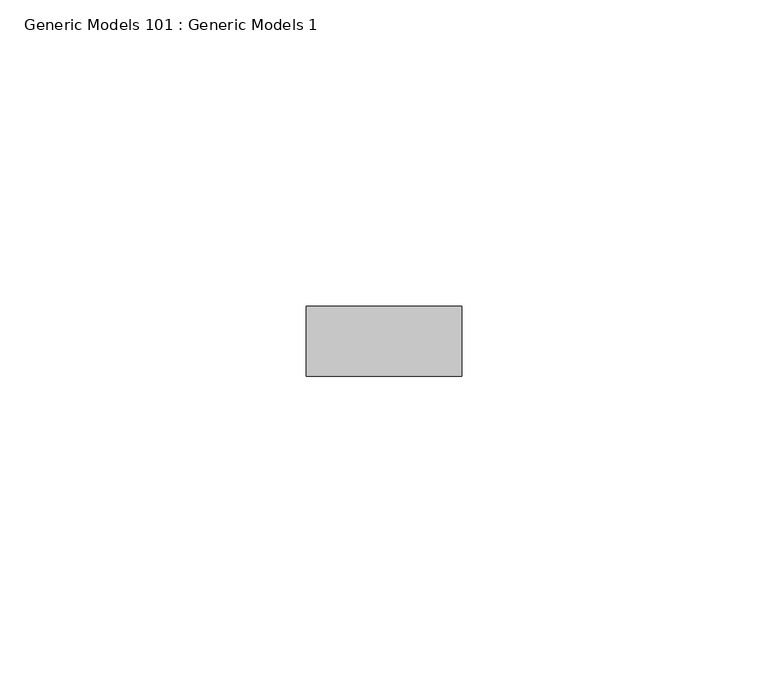
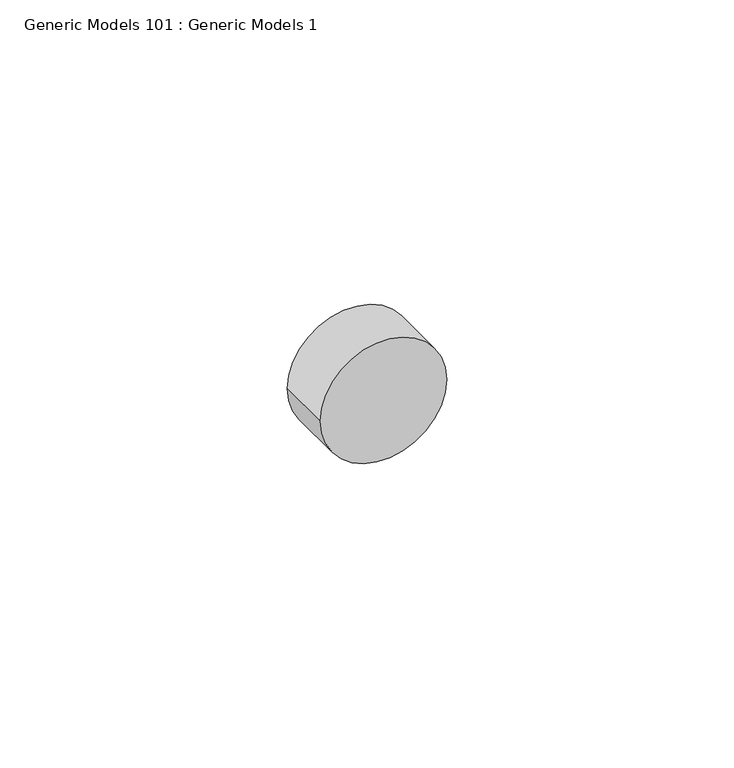
"""IFC4 building model written with IfcOpenShell, lengths in millimetres: proxy geometry, Generic Models 101 : Generic Models 1."""

import ifcopenshell
import ifcopenshell.guid

model = None  # the IFC model being written
_history = None  # IfcOwnerHistory: only IFC2X3 demands one
_inside = {}  # id of a spatial element -> (the spatial element, [elements in it])
_under = {}  # id of a project, library or spatial element -> (it, [spatial elements below it])
_declared = {}  # id of a project -> (the project, [libraries it declares])
_typed = {}  # id of a type object -> (the type object, [elements of that type])
_made_of = {}  # id of a material, layer set ... -> (it, [elements and type objects made of it])


def new_model(schema):
    """Start an empty IFC model of exactly this schema.

    Asked for "IFC4X3", IfcOpenShell would pick the latest addendum, in which some entities
    have other attributes; the version numbers below select the first issue.
    IFC2X3 requires an IfcOwnerHistory on every rooted entity: one is made here for all.
    """
    global model, _history
    if schema == "IFC4X3":
        model = ifcopenshell.file(schema_version=(4, 3, 0, 0))
    else:
        model = ifcopenshell.file(schema=schema)
    _inside.clear()
    _under.clear()
    _declared.clear()
    _typed.clear()
    _made_of.clear()
    _history = None
    if model.schema == "IFC2X3":
        org = make("IfcOrganization", Name="unknown")
        user = make(
            "IfcPersonAndOrganization",
            ThePerson=make("IfcPerson", FamilyName="unknown"),
            TheOrganization=org,
        )
        app = make(
            "IfcApplication",
            ApplicationDeveloper=org,
            Version="unknown",
            ApplicationFullName="unknown",
            ApplicationIdentifier="unknown",
        )
        _history = make(
            "IfcOwnerHistory",
            OwningUser=user,
            OwningApplication=app,
            ChangeAction="ADDED",
            CreationDate=0,
        )
    return model


def make(cls, **values):
    """One entity of the class cls with the attributes given. An attribute that is None is left unset."""
    return model.create_entity(
        cls, **{name: value for name, value in values.items() if value is not None}
    )


def rooted(cls, **values):
    """An entity with a GlobalId (a new one), such as an element, a storey or a relation."""
    return make(cls, GlobalId=ifcopenshell.guid.new(), OwnerHistory=_history, **values)


def si_unit(unit_type, name, prefix=None):
    """IfcSIUnit, for example si_unit("LENGTHUNIT", "METRE", prefix="MILLI")."""
    return make("IfcSIUnit", UnitType=unit_type, Prefix=prefix, Name=name)


def assignment(units):
    """IfcUnitAssignment: the units of a project."""
    return None if units is None else make("IfcUnitAssignment", Units=units)


def point(xyz):
    """IfcCartesianPoint."""
    return None if xyz is None else make("IfcCartesianPoint", Coordinates=xyz)


def direction(xyz):
    """IfcDirection."""
    return None if xyz is None else make("IfcDirection", DirectionRatios=xyz)


def frame(location, z_axis=None, x_axis=None):
    """IfcAxis2Placement3D, a coordinate frame: its origin and axes. An axis left out is left unset."""
    return make(
        "IfcAxis2Placement3D",
        Location=point(location),
        Axis=direction(z_axis),
        RefDirection=direction(x_axis),
    )


def frame_2d(location, x_axis=None):
    """IfcAxis2Placement2D, a coordinate frame in the plane: its origin and x axis."""
    return make(
        "IfcAxis2Placement2D", Location=point(location), RefDirection=direction(x_axis)
    )


def origin():
    """The frame at (0, 0, 0) with its axes left unset."""
    return frame((0.0, 0.0, 0.0))


def place(relative_to, where):
    """IfcLocalPlacement: puts the frame where relative to a parent placement (None: the world)."""
    return make(
        "IfcLocalPlacement", PlacementRelTo=relative_to, RelativePlacement=where
    )


def context(
    kind, dimensions, precision=None, world=None, true_north=None, identifier=None
):
    """IfcGeometricRepresentationContext, for example the 3D "Model" context."""
    return make(
        "IfcGeometricRepresentationContext",
        ContextIdentifier=identifier,
        ContextType=kind,
        CoordinateSpaceDimension=dimensions,
        Precision=precision,
        WorldCoordinateSystem=world,
        TrueNorth=true_north,
    )


def project(units=None, contexts=None):
    """IfcProject with its units and contexts."""
    return rooted(
        "IfcProject",
        Name="project",
        RepresentationContexts=contexts,
        UnitsInContext=assignment(units),
    )


def spatial(cls, under=None, at=None, **own):
    """A site, building, storey or space (cls), placed at a placement, below another one or the project."""
    s = rooted(cls, ObjectPlacement=at, **own)
    if under is not None:
        _under.setdefault(under.id(), (under, []))[1].append(s)
    return s


def circle_curve(where, radius):
    """IfcCircle in the frame where."""
    return make("IfcCircle", Position=where, Radius=radius)


def trimmed(basis, trim1, trim2, sense, master):
    """IfcTrimmedCurve: the piece of a basis curve between two trims."""
    return make(
        "IfcTrimmedCurve",
        BasisCurve=basis,
        Trim1=trim1,
        Trim2=trim2,
        SenseAgreement=sense,
        MasterRepresentation=master,
    )


def segment(curve, same_sense, transition):
    """IfcCompositeCurveSegment."""
    return make(
        "IfcCompositeCurveSegment",
        Transition=transition,
        SameSense=same_sense,
        ParentCurve=curve,
    )


def composite_curve(segments, self_intersect=None):
    """IfcCompositeCurve: segments joined end to end."""
    return make("IfcCompositeCurve", Segments=segments, SelfIntersect=self_intersect)


def outline(outer, holes=None, kind="AREA"):
    """IfcArbitraryClosedProfileDef: a profile drawn as a closed curve; with holes, ...WithVoids."""
    if holes is None:
        return make("IfcArbitraryClosedProfileDef", ProfileType=kind, OuterCurve=outer)
    return make(
        "IfcArbitraryProfileDefWithVoids",
        ProfileType=kind,
        OuterCurve=outer,
        InnerCurves=holes,
    )


def extrude(swept, where, along, depth):
    """IfcExtrudedAreaSolid: the profile swept, set in the frame where, extruded along a direction by depth."""
    return make(
        "IfcExtrudedAreaSolid",
        SweptArea=swept,
        Position=where,
        ExtrudedDirection=direction(along),
        Depth=depth,
    )


def shape(context_of_items, identifier, shape_type, items):
    """IfcShapeRepresentation: the items that make up one representation, for example the "Body"."""
    return make(
        "IfcShapeRepresentation",
        ContextOfItems=context_of_items,
        RepresentationIdentifier=identifier,
        RepresentationType=shape_type,
        Items=items,
    )


def source(mapping_origin, context_of_items, identifier, shape_type, items):
    """IfcRepresentationMap: a shape defined once, which mapped items show again and again."""
    return make(
        "IfcRepresentationMap",
        MappingOrigin=mapping_origin,
        MappedRepresentation=shape(context_of_items, identifier, shape_type, items),
    )


def transform(
    local_origin,
    x_axis=None,
    y_axis=None,
    z_axis=None,
    scale=None,
    scale2=None,
    scale3=None,
    uniform=True,
):
    """IfcCartesianTransformationOperator3D, or its non-uniform kind. x_axis, y_axis, z_axis: its Axis1, 2, 3."""
    if uniform:
        return make(
            "IfcCartesianTransformationOperator3D",
            Axis1=direction(x_axis),
            Axis2=direction(y_axis),
            LocalOrigin=point(local_origin),
            Scale=scale,
            Axis3=direction(z_axis),
        )
    return make(
        "IfcCartesianTransformationOperator3DnonUniform",
        Axis1=direction(x_axis),
        Axis2=direction(y_axis),
        LocalOrigin=point(local_origin),
        Scale=scale,
        Axis3=direction(z_axis),
        Scale2=scale2,
        Scale3=scale3,
    )


def mapped(mapping_source, mapping_target):
    """IfcMappedItem: shows the shape of a source again, moved by a transform."""
    return make(
        "IfcMappedItem", MappingSource=mapping_source, MappingTarget=mapping_target
    )


def made_of(thing, what):
    """Note that an element or type object is made of a material, layer set ...; save() writes the relation."""
    if what is not None:
        _made_of.setdefault(what.id(), (what, []))[1].append(thing)
    return thing


def element(
    cls,
    number,
    at=None,
    inside=None,
    cuts=None,
    type_object=None,
    material=None,
    context=None,
    identifier="Body",
    shape_type=None,
    held_by="IfcProductDefinitionShape",
    body=None,
    shapes=None,
    **own,
):
    """One element of the class cls, such as IfcWall. Its Tag is "e" and its number.

    at: its placement. inside: the storey or other place that contains it. cuts: it is an
    opening in that element (IfcRelVoidsElement). A single representation is given by context,
    identifier, shape_type and body (its items); several are given by shapes. held_by: the class
    of the entity that holds the representations. save() writes the other relations.
    """
    e = rooted(cls, Tag="e%d" % number, ObjectPlacement=at, **own)
    if body is not None:
        shapes = [shape(context, identifier, shape_type, body)]
    if shapes is not None:
        e.Representation = make(held_by, Representations=shapes)
    if inside is not None:
        _inside.setdefault(inside.id(), (inside, []))[1].append(e)
    if cuts is not None:
        rooted(
            "IfcRelVoidsElement", RelatingBuildingElement=cuts, RelatedOpeningElement=e
        )
    if type_object is not None:
        _typed.setdefault(type_object.id(), (type_object, []))[1].append(e)
    return made_of(e, material)


def aggregate(whole, parts):
    """IfcRelAggregates: a whole, such as a stair, and the parts it consists of."""
    return rooted("IfcRelAggregates", RelatingObject=whole, RelatedObjects=parts)


def save(model, path):
    """Write the relations noted so far, then the file.

    IfcRelAggregates (storeys below a building ...), IfcRelContainedInSpatialStructure (elements
    in a storey), IfcRelDefinesByType, IfcRelAssociatesMaterial and IfcRelDeclares: one each for
    every whole, place, type object, material and project.
    """
    for whole, parts in _under.values():
        aggregate(whole, parts)
    for where, things in _inside.values():
        rooted(
            "IfcRelContainedInSpatialStructure",
            RelatedElements=things,
            RelatingStructure=where,
        )
    for kind, things in _typed.values():
        rooted("IfcRelDefinesByType", RelatedObjects=things, RelatingType=kind)
    for what, things in _made_of.values():
        rooted("IfcRelAssociatesMaterial", RelatedObjects=things, RelatingMaterial=what)
    for by, libraries in _declared.values():
        rooted("IfcRelDeclares", RelatingContext=by, RelatedDefinitions=libraries)
    model.write(path)


def generic_models_101_generic_models_1_eaa3b5e4(model_context):
    return source(origin(), model_context, "Body", "SweptSolid", [
        extrude(outline(composite_curve([segment(trimmed(circle_curve(frame_2d((37345.8776334, 6010.5828124)), 12.7), [point((37345.8776334, 5997.8828124))], [point((37345.8776334, 6023.2828124))], False, "CARTESIAN"), True, "CONTINUOUS"), segment(trimmed(circle_curve(frame_2d((37345.8776334, 6010.5828124)), 12.7), [point((37345.8776334, 6023.2828124))], [point((37345.8776334, 5997.8828124))], False, "CARTESIAN"), True, "CONTINUOUS")], self_intersect=False)), frame((0.0, 1836.9202358, 0.0), z_axis=(0.0, 1.0, 0.0), x_axis=(0.0, 0.0, 1.0)), (0.0, 0.0, 1.0), 11.4464372),
    ])


if __name__ == "__main__":
    model = new_model("IFC4")
    model_context = context("Model", 3, world=origin())
    ifc_project = project(units=[si_unit("LENGTHUNIT", "METRE", prefix="MILLI")], contexts=[model_context])
    site = spatial("IfcSite", under=ifc_project)
    building = spatial("IfcBuilding", under=site)
    placement = place(None, origin())
    generic_models_101_generic_models_1_shape = generic_models_101_generic_models_1_eaa3b5e4(model_context)
    element("IfcBuildingElementProxy", 1, Name="Generic Models 101 : Generic Models 1", ObjectType="Generic Models 101 : Generic Models 1", at=placement, inside=building, context=model_context, shape_type="MappedRepresentation", body=[
        mapped(generic_models_101_generic_models_1_shape, transform((0.0, 0.0, 0.0), x_axis=(1.0, 0.0, 0.0), y_axis=(0.0, 1.0, 0.0), z_axis=(0.0, 0.0, 1.0))),
    ])
    save(model, "model.ifc")

# Revit data of these elements
# Element 1 (IfcBuildingElementProxy, "Generic Models 101 : Generic Models 1")
#   Materials on its faces: "S.S. LAG BOLT - SEE STRUCT. DWGS"
# Materials
#   "S.S. LAG BOLT - SEE STRUCT. DWGS": class "Generic", colour RGB 120 120 120, transparency 0, Cost = 0
